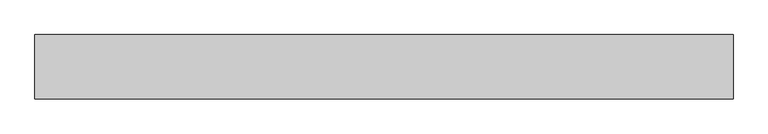
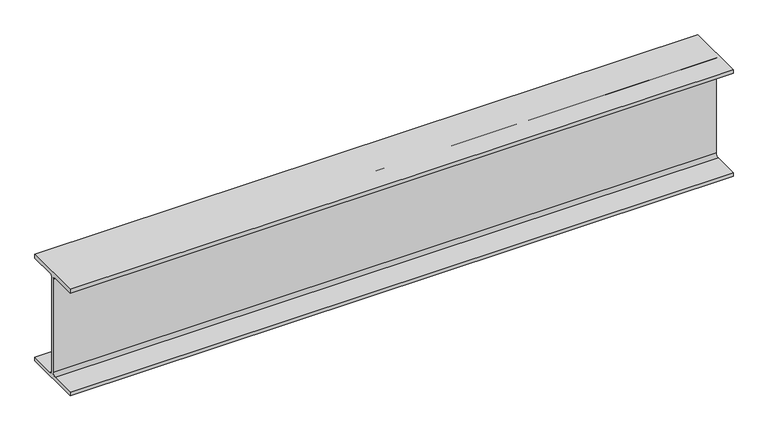
"""IFC4 building model written with IfcOpenShell, lengths in millimetres: beam geometry, Old_Steel Beam_H-KSD3502 : H_SB_ASB_H-200×200x8x12."""

from ifc_helpers import new_model, si_unit, point, frame, frame_2d, origin, place, context, project, spatial, polyline, circle_curve, trimmed, segment, composite_curve, outline, extrude, source, transform, mapped, element, save


def beam_f43078d7(model_context):
    return source(origin(), model_context, "Body", "SweptSolid", [
        extrude(outline(composite_curve([segment(polyline([(82.5, -141.5), (82.5, -151.7), (-82.5, -151.7), (-82.5, -141.5), (-11.9, -141.5)]), True, "CONTINUOUS"), segment(trimmed(circle_curve(frame_2d((-11.9, -132.6)), 8.9), [point((-11.9, -141.5))], [point((-3.0, -132.6))], True, "CARTESIAN"), True, "CONTINUOUS"), segment(polyline([(-3.0, -132.6), (-3.0, 132.6)]), True, "CONTINUOUS"), segment(trimmed(circle_curve(frame_2d((-11.9, 132.6)), 8.9), [point((-3.0, 132.6))], [point((-11.9, 141.5))], True, "CARTESIAN"), True, "CONTINUOUS"), segment(polyline([(-11.9, 141.5), (-82.5, 141.5), (-82.5, 151.7), (82.5, 151.7), (82.5, 141.5), (11.9, 141.5)]), True, "CONTINUOUS"), segment(trimmed(circle_curve(frame_2d((11.9, 132.6)), 8.9), [point((11.9, 141.5))], [point((3.0, 132.6))], True, "CARTESIAN"), True, "CONTINUOUS"), segment(polyline([(3.0, 132.6), (3.0, -132.6)]), True, "CONTINUOUS"), segment(trimmed(circle_curve(frame_2d((11.9, -132.6)), 8.9), [point((3.0, -132.6))], [point((11.9, -141.5))], True, "CARTESIAN"), True, "CONTINUOUS"), segment(polyline([(11.9, -141.5), (82.5, -141.5)]), True, "CONTINUOUS")], self_intersect=False)), frame((-822.025694, 0.0, 0.0), z_axis=(1.0, 0.0, 0.0), x_axis=(0.0, 1.0, 0.0)), (0.0, 0.0, 1.0), 1791.5376517),
    ])


if __name__ == "__main__":
    model = new_model("IFC4")
    model_context = context("Model", 3, world=origin())
    ifc_project = project(units=[si_unit("LENGTHUNIT", "METRE", prefix="MILLI")], contexts=[model_context])
    site = spatial("IfcSite", under=ifc_project)
    building = spatial("IfcBuilding", under=site)
    placement = place(None, origin())
    beam_shape = beam_f43078d7(model_context)
    element("IfcBeam", 1, ObjectType="Old_Steel Beam_H-KSD3502 : H_SB_ASB_H-200×200x8x12", at=placement, inside=building, context=model_context, shape_type="MappedRepresentation", body=[
        mapped(beam_shape, transform((0.0, 0.0, 0.0), x_axis=(1.0, 0.0, 0.0), y_axis=(0.0, 1.0, 0.0), z_axis=(0.0, 0.0, 1.0))),
    ])
    save(model, "model.ifc")

# Revit data of these elements
# Type "Old_Steel Beam_H-KSD3502 : H_SB_ASB_H-200×200x8x12"
#   Width = 20.0 cm
#   Web Thickness = 0.8 cm
#   Web Fillet = 1.3 cm
#   Warping Constant = 141376.0 cm⁶
#   Torsional Moment of Inertia = 26.2485 cm⁴
#   Torsional Modulus = 1.0 cm³
#   Section Area = 63.53 cm²
#   Plastic Modulus weak axis = 244.0 cm³
#   Plastic Modulus strong axis = 525.0 cm³
#   Perimeter = 1.16 m²/m
#   Nominal Weight = 49.90 kgf/m
#   Moment of Inertia weak axis = 1600.00 cm⁴
#   Moment of Inertia strong axis = 4720.00 cm⁴
#   Height = 20.0 cm
#   Flange Thickness = 1.2 cm
#   Elastic Modulus weak axis = 160.0 cm³
#   Elastic Modulus strong axis = 472.0 cm³
#   Centroid Vertical = 10.0 cm
#   Centroid Horizontal = 10.0 cm
#   Length [instance default] = 1.5240 m
#   Structural Material [instance default] = Steel, 45-345
#   Assembly Code = ""
# Element 1 (IfcBeam, "Old_Steel Beam_H-KSD3502 : H_SB_ASB_H-200×200x8x12")
#   Structural Material = none
# Materials
#   "Steel, 45-345": class "Metal", colour RGB 189 187 185, transparency 0, Description = "Steel 345 MPa", Cost = 0
